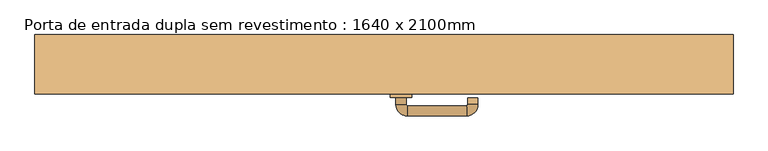
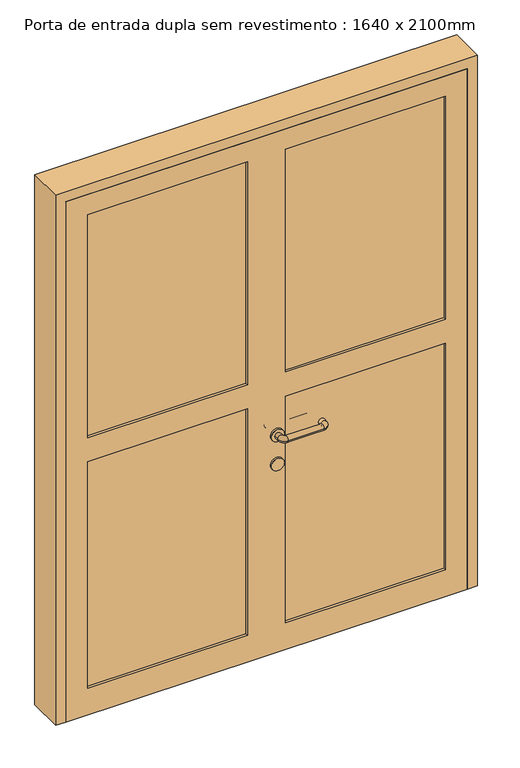
"""IFC4 building model written with IfcOpenShell, lengths in millimetres: door geometry, Porta de entrada dupla sem revestimento : 1640 x 2100mm."""

from ifc_helpers import new_model, si_unit, point, frame, frame_2d, origin, place, context, project, spatial, polyline, circle_curve, ellipse_curve, trimmed, segment, composite_curve, outline, extrude, faceted_brep, source, transform, mapped, element, save
from ifc_brep_helpers import plane_surface, cylinder_surface, revolved_surface, advanced_brep


def porta_de_entrada_dupla_sem_revestimento_1640_x_2100mm_88b676f1(model_context):
    return source(origin(), model_context, "Body", "SolidModel", [
        advanced_brep(
        [(52.0, -27.0, 900.0), (28.0, -27.0, 900.0), (52.0, -10.0, 900.0), (28.0, -10.0, 900.0), (55.0, 17.0, 900.0), (55.0, -7.0, 900.0), (195.0, -7.0, 900.0), (195.0, 17.0, 900.0), (222.0, -10.0, 900.0), (198.0, -10.0, 900.0), (198.0, -25.0, 900.0), (222.0, -25.0, 900.0)],
        [
            (0, 1, circle_curve(frame((40.0, -27.0, 900.0), z_axis=(0.0, -1.0, 0.0), x_axis=(-1.0, 0.0, 0.0)), 12.0)),
            (1, 0, circle_curve(frame((40.0, -27.0, 900.0), z_axis=(0.0, -1.0, 0.0), x_axis=(-1.0, 0.0, 0.0)), 12.0)),
            (0, 2),
            (2, 3, circle_curve(frame((40.0, -10.0, 900.0), z_axis=(0.0, -1.0, 0.0), x_axis=(-1.0, 0.0, 0.0)), 12.0)),
            (3, 1),
            (3, 2, circle_curve(frame((40.0, -10.0, 900.0), z_axis=(0.0, -1.0, 0.0), x_axis=(-1.0, 0.0, 0.0)), 12.0)),
            (4, 3, circle_curve(frame((55.0, -10.0, 900.0), z_axis=(0.0, 0.0, 1.0), x_axis=(-1.0, 0.0, 0.0)), 27.0)),
            (2, 5, circle_curve(frame((55.0, -10.0, 900.0), z_axis=(0.0, 0.0, -1.0), x_axis=(-1.0, 0.0, 0.0)), 3.0)),
            (5, 4, circle_curve(frame((55.0, 5.0, 900.0), z_axis=(-1.0, 0.0, 0.0), x_axis=(0.0, 1.0, 0.0)), 12.0)),
            (4, 5, circle_curve(frame((55.0, 5.0, 900.0), z_axis=(-1.0, 0.0, 0.0), x_axis=(0.0, 1.0, 0.0)), 12.0)),
            (5, 6),
            (6, 7, circle_curve(frame((195.0, 5.0, 900.0), z_axis=(-1.0, 0.0, 0.0), x_axis=(0.0, 1.0, 0.0)), 12.0)),
            (7, 4),
            (7, 6, circle_curve(frame((195.0, 5.0, 900.0), z_axis=(-1.0, 0.0, 0.0), x_axis=(0.0, 1.0, 0.0)), 12.0)),
            (8, 7, circle_curve(frame((195.0, -10.0, 900.0), z_axis=(0.0, 0.0, 1.0), x_axis=(0.0, 1.0, 0.0)), 27.0)),
            (6, 9, circle_curve(frame((195.0, -10.0, 900.0), z_axis=(0.0, 0.0, -1.0), x_axis=(0.0, 1.0, 0.0)), 3.0)),
            (9, 8, circle_curve(frame((210.0, -10.0, 900.0), z_axis=(0.0, 1.0, 0.0), x_axis=(1.0, 0.0, 0.0)), 12.0)),
            (8, 9, circle_curve(frame((210.0, -10.0, 900.0), z_axis=(0.0, 1.0, 0.0), x_axis=(1.0, 0.0, 0.0)), 12.0)),
            (10, 11, circle_curve(frame((210.0, -25.0, 900.0), z_axis=(0.0, -1.0, 0.0), x_axis=(1.0, 0.0, 0.0)), 12.0)),
            (11, 10, circle_curve(frame((210.0, -25.0, 900.0), z_axis=(0.0, -1.0, 0.0), x_axis=(1.0, 0.0, 0.0)), 12.0)),
            (9, 10),
            (11, 8),
        ],
        [
            plane_surface(frame((-802.0, -27.0, 1730.0), z_axis=(0.0, -1.0, 0.0), x_axis=(0.0, 0.0, 1.0))),
            cylinder_surface(frame((40.0, -27.0, 900.0), z_axis=(0.0, -1.0, 0.0), x_axis=(-1.0, 0.0, 0.0)), 12.0),
            revolved_surface(trimmed(ellipse_curve(frame((40.0, -10.0, 900.0), z_axis=(0.0, -1.0, 0.0), x_axis=(-1.0, 0.0, 0.0)), 12.0, 12.0), [point((52.0, -10.0, 900.0))], [point((28.0, -10.0, 900.0))], True, "CARTESIAN"), (55.0, -10.0, 1730.0), (0.0, 0.0, -1.0)),
            revolved_surface(trimmed(ellipse_curve(frame((40.0, -10.0, 900.0), z_axis=(0.0, -1.0, 0.0), x_axis=(-1.0, 0.0, 0.0)), 12.0, 12.0), [point((28.0, -10.0, 900.0))], [point((52.0, -10.0, 900.0))], True, "CARTESIAN"), (55.0, -10.0, 1730.0), (0.0, 0.0, -1.0)),
            cylinder_surface(frame((55.0, 5.0, 900.0), z_axis=(-1.0, 0.0, 0.0), x_axis=(0.0, 1.0, 0.0)), 12.0),
            revolved_surface(trimmed(ellipse_curve(frame((195.0, 5.0, 900.0), z_axis=(-1.0, 0.0, 0.0), x_axis=(0.0, 1.0, 0.0)), 12.0, 12.0), [point((195.0, -7.0, 900.0))], [point((195.0, 17.0, 900.0))], True, "CARTESIAN"), (195.0, -10.0, 1730.0), (0.0, 0.0, -1.0)),
            revolved_surface(trimmed(ellipse_curve(frame((195.0, 5.0, 900.0), z_axis=(-1.0, 0.0, 0.0), x_axis=(0.0, 1.0, 0.0)), 12.0, 12.0), [point((195.0, 17.0, 900.0))], [point((195.0, -7.0, 900.0))], True, "CARTESIAN"), (195.0, -10.0, 1730.0), (0.0, 0.0, -1.0)),
            plane_surface(frame((-632.0, -25.0, 1730.0), z_axis=(0.0, -1.0, 0.0), x_axis=(0.0, 0.0, -1.0))),
            cylinder_surface(frame((210.0, -10.0, 900.0), z_axis=(0.0, 1.0, 0.0), x_axis=(1.0, 0.0, 0.0)), 12.0),
        ],
        [
            (0, [[1, 2]]),
            (1, [[-1, 3, 4, 5]]),
            (1, [[-2, -5, 6, -3]]),
            (2, [[7, -4, 8, 9]]),
            (3, [[-8, -6, -7, 10]]),
            (4, [[-9, 11, 12, 13]]),
            (4, [[-10, -13, 14, -11]]),
            (5, [[15, -12, 16, 17]]),
            (6, [[-16, -14, -15, 18]]),
            (7, [[19, 20]]),
            (8, [[-17, 21, -20, 22]]),
            (8, [[-18, -22, -19, -21]]),
        ],
    ),
        extrude(outline(composite_curve([segment(trimmed(circle_curve(frame_2d((780.0, 40.0)), 25.0), [point((780.0, 15.0))], [point((780.0, 65.0))], False, "CARTESIAN"), True, "CONTINUOUS"), segment(trimmed(circle_curve(frame_2d((780.0, 40.0)), 25.0), [point((780.0, 65.0))], [point((780.0, 15.0))], False, "CARTESIAN"), True, "CONTINUOUS")], self_intersect=False)), frame((0.0, -35.0, 0.0), z_axis=(0.0, 1.0, 0.0), x_axis=(0.0, 0.0, 1.0)), (0.0, 0.0, 1.0), 8.0),
        extrude(outline(composite_curve([segment(trimmed(circle_curve(frame_2d((900.0, 40.0)), 25.0), [point((900.0, 15.0))], [point((900.0, 65.0))], False, "CARTESIAN"), True, "CONTINUOUS"), segment(trimmed(circle_curve(frame_2d((900.0, 40.0)), 25.0), [point((900.0, 65.0))], [point((900.0, 15.0))], False, "CARTESIAN"), True, "CONTINUOUS")], self_intersect=False)), frame((0.0, -35.0, 0.0), z_axis=(0.0, 1.0, 0.0), x_axis=(0.0, 0.0, 1.0)), (0.0, 0.0, 1.0), 8.0),
        advanced_brep(
        [(28.0, -78.0, 900.0), (52.0, -78.0, 900.0), (28.0, -95.0, 900.0), (52.0, -95.0, 900.0), (55.0, -98.0, 900.0), (55.0, -122.0, 900.0), (195.0, -122.0, 900.0), (195.0, -98.0, 900.0), (198.0, -95.0, 900.0), (222.0, -95.0, 900.0), (222.0, -80.0, 900.0), (198.0, -80.0, 900.0)],
        [
            (0, 1, circle_curve(frame((40.0, -78.0, 900.0), z_axis=(0.0, 1.0, 0.0), x_axis=(1.0, 0.0, 0.0)), 12.0)),
            (1, 0, circle_curve(frame((40.0, -78.0, 900.0), z_axis=(0.0, 1.0, 0.0), x_axis=(1.0, 0.0, 0.0)), 12.0)),
            (0, 2),
            (2, 3, circle_curve(frame((40.0, -95.0, 900.0), z_axis=(0.0, 1.0, 0.0), x_axis=(1.0, 0.0, 0.0)), 12.0)),
            (3, 1),
            (3, 2, circle_curve(frame((40.0, -95.0, 900.0), z_axis=(0.0, 1.0, 0.0), x_axis=(1.0, 0.0, 0.0)), 12.0)),
            (4, 3, circle_curve(frame((55.0, -95.0, 900.0), z_axis=(0.0, 0.0, -1.0), x_axis=(-1.0, 0.0, 0.0)), 3.0)),
            (2, 5, circle_curve(frame((55.0, -95.0, 900.0), z_axis=(0.0, 0.0, 1.0), x_axis=(-1.0, 0.0, 0.0)), 27.0)),
            (5, 4, circle_curve(frame((55.0, -110.0, 900.0), z_axis=(-1.0, 0.0, 0.0), x_axis=(0.0, 1.0, 0.0)), 12.0)),
            (4, 5, circle_curve(frame((55.0, -110.0, 900.0), z_axis=(-1.0, 0.0, 0.0), x_axis=(0.0, 1.0, 0.0)), 12.0)),
            (5, 6),
            (6, 7, circle_curve(frame((195.0, -110.0, 900.0), z_axis=(-1.0, 0.0, 0.0), x_axis=(0.0, 1.0, 0.0)), 12.0)),
            (7, 4),
            (7, 6, circle_curve(frame((195.0, -110.0, 900.0), z_axis=(-1.0, 0.0, 0.0), x_axis=(0.0, 1.0, 0.0)), 12.0)),
            (8, 7, circle_curve(frame((195.0, -95.0, 900.0), z_axis=(0.0, 0.0, -1.0), x_axis=(0.0, -1.0, 0.0)), 3.0)),
            (6, 9, circle_curve(frame((195.0, -95.0, 900.0), z_axis=(0.0, 0.0, 1.0), x_axis=(0.0, -1.0, 0.0)), 27.0)),
            (9, 8, circle_curve(frame((210.0, -95.0, 900.0), z_axis=(0.0, -1.0, 0.0), x_axis=(-1.0, 0.0, 0.0)), 12.0)),
            (8, 9, circle_curve(frame((210.0, -95.0, 900.0), z_axis=(0.0, -1.0, 0.0), x_axis=(-1.0, 0.0, 0.0)), 12.0)),
            (10, 11, circle_curve(frame((210.0, -80.0, 900.0), z_axis=(0.0, 1.0, 0.0), x_axis=(-1.0, 0.0, 0.0)), 12.0)),
            (11, 10, circle_curve(frame((210.0, -80.0, 900.0), z_axis=(0.0, 1.0, 0.0), x_axis=(-1.0, 0.0, 0.0)), 12.0)),
            (9, 10),
            (11, 8),
        ],
        [
            plane_surface(frame((-802.0, -78.0, 1730.0), z_axis=(0.0, 1.0, 0.0), x_axis=(0.0, 0.0, -1.0))),
            cylinder_surface(frame((40.0, -78.0, 900.0), z_axis=(0.0, 1.0, 0.0), x_axis=(1.0, 0.0, 0.0)), 12.0),
            revolved_surface(trimmed(ellipse_curve(frame((40.0, -95.0, 900.0), z_axis=(0.0, 1.0, 0.0), x_axis=(1.0, 0.0, 0.0)), 12.0, 12.0), [point((28.0, -95.0, 900.0))], [point((52.0, -95.0, 900.0))], True, "CARTESIAN"), (55.0, -95.0, 1730.0), (0.0, 0.0, 1.0)),
            revolved_surface(trimmed(ellipse_curve(frame((40.0, -95.0, 900.0), z_axis=(0.0, 1.0, 0.0), x_axis=(1.0, 0.0, 0.0)), 12.0, 12.0), [point((52.0, -95.0, 900.0))], [point((28.0, -95.0, 900.0))], True, "CARTESIAN"), (55.0, -95.0, 1730.0), (0.0, 0.0, 1.0)),
            cylinder_surface(frame((55.0, -110.0, 900.0), z_axis=(-1.0, 0.0, 0.0), x_axis=(0.0, 1.0, 0.0)), 12.0),
            revolved_surface(trimmed(ellipse_curve(frame((195.0, -110.0, 900.0), z_axis=(-1.0, 0.0, 0.0), x_axis=(0.0, 1.0, 0.0)), 12.0, 12.0), [point((195.0, -122.0, 900.0))], [point((195.0, -98.0, 900.0))], True, "CARTESIAN"), (195.0, -95.0, 1730.0), (0.0, 0.0, 1.0)),
            revolved_surface(trimmed(ellipse_curve(frame((195.0, -110.0, 900.0), z_axis=(-1.0, 0.0, 0.0), x_axis=(0.0, 1.0, 0.0)), 12.0, 12.0), [point((195.0, -98.0, 900.0))], [point((195.0, -122.0, 900.0))], True, "CARTESIAN"), (195.0, -95.0, 1730.0), (0.0, 0.0, 1.0)),
            plane_surface(frame((-632.0, -80.0, 1730.0), z_axis=(0.0, 1.0, 0.0), x_axis=(0.0, 0.0, 1.0))),
            cylinder_surface(frame((210.0, -95.0, 900.0), z_axis=(0.0, -1.0, 0.0), x_axis=(-1.0, 0.0, 0.0)), 12.0),
        ],
        [
            (0, [[1, 2]]),
            (1, [[-1, 3, 4, 5]]),
            (1, [[-2, -5, 6, -3]]),
            (2, [[7, -4, 8, 9]]),
            (3, [[-8, -6, -7, 10]]),
            (4, [[-9, 11, 12, 13]]),
            (4, [[-10, -13, 14, -11]]),
            (5, [[15, -12, 16, 17]]),
            (6, [[-16, -14, -15, 18]]),
            (7, [[19, 20]]),
            (8, [[-17, 21, -20, 22]]),
            (8, [[-18, -22, -19, -21]]),
        ],
    ),
        extrude(outline(composite_curve([segment(trimmed(circle_curve(frame_2d((780.0, 40.0)), 25.0), [point((780.0, 15.0))], [point((780.0, 65.0))], False, "CARTESIAN"), True, "CONTINUOUS"), segment(trimmed(circle_curve(frame_2d((780.0, 40.0)), 25.0), [point((780.0, 65.0))], [point((780.0, 15.0))], False, "CARTESIAN"), True, "CONTINUOUS")], self_intersect=False)), frame((0.0, -78.0, 0.0), z_axis=(0.0, 1.0, 0.0), x_axis=(0.0, 0.0, 1.0)), (0.0, 0.0, 1.0), 8.0),
        extrude(outline(composite_curve([segment(trimmed(circle_curve(frame_2d((900.0, 40.0)), 25.0), [point((900.0, 15.0))], [point((900.0, 65.0))], False, "CARTESIAN"), True, "CONTINUOUS"), segment(trimmed(circle_curve(frame_2d((900.0, 40.0)), 25.0), [point((900.0, 65.0))], [point((900.0, 15.0))], False, "CARTESIAN"), True, "CONTINUOUS")], self_intersect=False)), frame((0.0, -78.0, 0.0), z_axis=(0.0, 1.0, 0.0), x_axis=(0.0, 0.0, 1.0)), (0.0, 0.0, 1.0), 8.0),
        extrude(outline(polyline([(-740.0, -45.5), (740.0, -45.5), (740.0, -59.5), (-740.0, -59.5), (-740.0, -45.5)])), frame((0.0, 0.0, 70.0), z_axis=(0.0, 0.0, 1.0), x_axis=(1.0, 0.0, 0.0)), (0.0, 0.0, 1.0), 1015.0),
        extrude(outline(polyline([(-740.0, -45.5), (740.0, -45.5), (740.0, -59.5), (-740.0, -59.5), (-740.0, -45.5)])), frame((0.0, 0.0, 1105.0), z_axis=(0.0, 0.0, 1.0), x_axis=(1.0, 0.0, 0.0)), (0.0, 0.0, 1.0), 1000.0),
        extrude(outline(polyline([(-740.0, -45.5), (740.0, -45.5), (740.0, -59.5), (-740.0, -59.5), (-740.0, -45.5)])), frame((0.0, 0.0, 70.0), z_axis=(0.0, 0.0, 1.0), x_axis=(1.0, 0.0, 0.0)), (0.0, 0.0, 1.0), 1015.0),
        extrude(outline(polyline([(-740.0, -45.5), (740.0, -45.5), (740.0, -59.5), (-740.0, -59.5), (-740.0, -45.5)])), frame((0.0, 0.0, 1105.0), z_axis=(0.0, 0.0, 1.0), x_axis=(1.0, 0.0, 0.0)), (0.0, 0.0, 1.0), 1000.0),
        faceted_brep([(-825.0, 70.0, 0.0), (-775.0, 70.0, 0.0), (-775.0, -32.0, 0.0), (-785.0, -32.0, 0.0), (-785.0, -70.0, 0.0), (-825.0, -70.0, 0.0), (-825.0, 70.0, 2190.0), (825.0, 70.0, 2190.0), (825.0, 70.0, 0.0), (775.0, 70.0, 0.0), (775.0, 70.0, 2140.0), (-775.0, 70.0, 2140.0), (-775.0, -32.0, 2140.0), (775.0, -32.0, 2140.0), (775.0, -32.0, 0.0), (785.0, -32.0, 0.0), (785.0, -32.0, 2150.0), (-785.0, -32.0, 2150.0), (-785.0, -70.0, 2150.0), (785.0, -70.0, 2150.0), (785.0, -70.0, 0.0), (825.0, -70.0, 0.0), (825.0, -70.0, 2190.0), (-825.0, -70.0, 2190.0)], [[[0, 1, 2, 3, 4, 5]], [[1, 0, 6, 7, 8, 9, 10, 11]], [[2, 1, 11, 12]], [[3, 2, 12, 13, 14, 15, 16, 17]], [[4, 3, 17, 18]], [[5, 4, 18, 19, 20, 21, 22, 23]], [[0, 5, 23, 6]], [[7, 22, 21, 8]], [[8, 21, 20, 15, 14, 9]], [[13, 10, 9, 14]], [[19, 16, 15, 20]], [[12, 11, 10, 13]], [[18, 17, 16, 19]], [[6, 23, 22, 7]]]),
        extrude(outline(polyline([(2150.0, -785.0), (0.0, -785.0), (0.0, 785.0), (2150.0, 785.0), (2150.0, -785.0)]), holes=[polyline([(2065.0, 75.0), (2065.0, 700.0), (1145.0, 700.0), (1145.0, 75.0), (2065.0, 75.0)]), polyline([(1145.0, -700.0), (2065.0, -700.0), (2065.0, -75.0), (1145.0, -75.0), (1145.0, -700.0)]), polyline([(1045.0, 700.0), (110.0, 700.0), (110.0, 75.0), (1045.0, 75.0), (1045.0, 700.0)]), polyline([(110.0, -75.0), (110.0, -700.0), (1045.0, -700.0), (1045.0, -75.0), (110.0, -75.0)])]), frame((0.0, -70.0, 0.0), z_axis=(0.0, 1.0, 0.0), x_axis=(0.0, 0.0, 1.0)), (0.0, 0.0, 1.0), 35.0),
    ])


if __name__ == "__main__":
    model = new_model("IFC4")
    model_context = context("Model", 3, world=origin())
    ifc_project = project(units=[si_unit("LENGTHUNIT", "METRE", prefix="MILLI")], contexts=[model_context])
    site = spatial("IfcSite", under=ifc_project)
    building = spatial("IfcBuilding", under=site)
    placement = place(None, origin())
    porta_de_entrada_dupla_sem_revestimento_1640_x_2100mm_shape = porta_de_entrada_dupla_sem_revestimento_1640_x_2100mm_88b676f1(model_context)
    element("IfcDoor", 1, ObjectType="Porta de entrada dupla sem revestimento : 1640 x 2100mm", at=placement, inside=building, context=model_context, shape_type="MappedRepresentation", body=[
        mapped(porta_de_entrada_dupla_sem_revestimento_1640_x_2100mm_shape, transform((0.0, 0.0, 0.0), x_axis=(1.0, 0.0, 0.0), y_axis=(0.0, 1.0, 0.0), z_axis=(0.0, 0.0, 1.0))),
    ])
    save(model, "model.ifc")

# Revit data of these elements
# Type "Porta de entrada dupla sem revestimento : 1640 x 2100mm"
#   Type Mark = "150"
#   Construction Type Id = "MPORTA"
#   Analytic Construction = "Metal"
#   W2 = 0.825 m
#   W1 = 1.570 m
#   Thickness = 0.035 m
#   Rough Width = 1.650 m
#   Rough Height = 2.190 m
#   Largura da moldura do painel = 0.075 m
#   Heat Transfer Coefficient (U) = 3.7021 W/(m²·K)
#   Largura da estrutura = 0.050 m
#   Height = 2.190 m
#   Width = 1.650 m
#   Define Thermal Properties by = 1
#   Function = 1
#   Material do painel = none
#   Material do puxador = none
#   Vidro = none
#   Material da moldura = none
#   Visual Light Transmittance = 0
#   Solar Heat Gain Coefficient = 0
#   Wall Closure = (empty or 0)
# Element 1 (IfcDoor, "Porta de entrada dupla sem revestimento : 1640 x 2100mm")
#   Materials on its faces: "Vidro 10mm"
# Materials
#   "Vidro 10mm": class "Glass", colour RGB 225 255 255, transparency 0.74, Cost = 0
